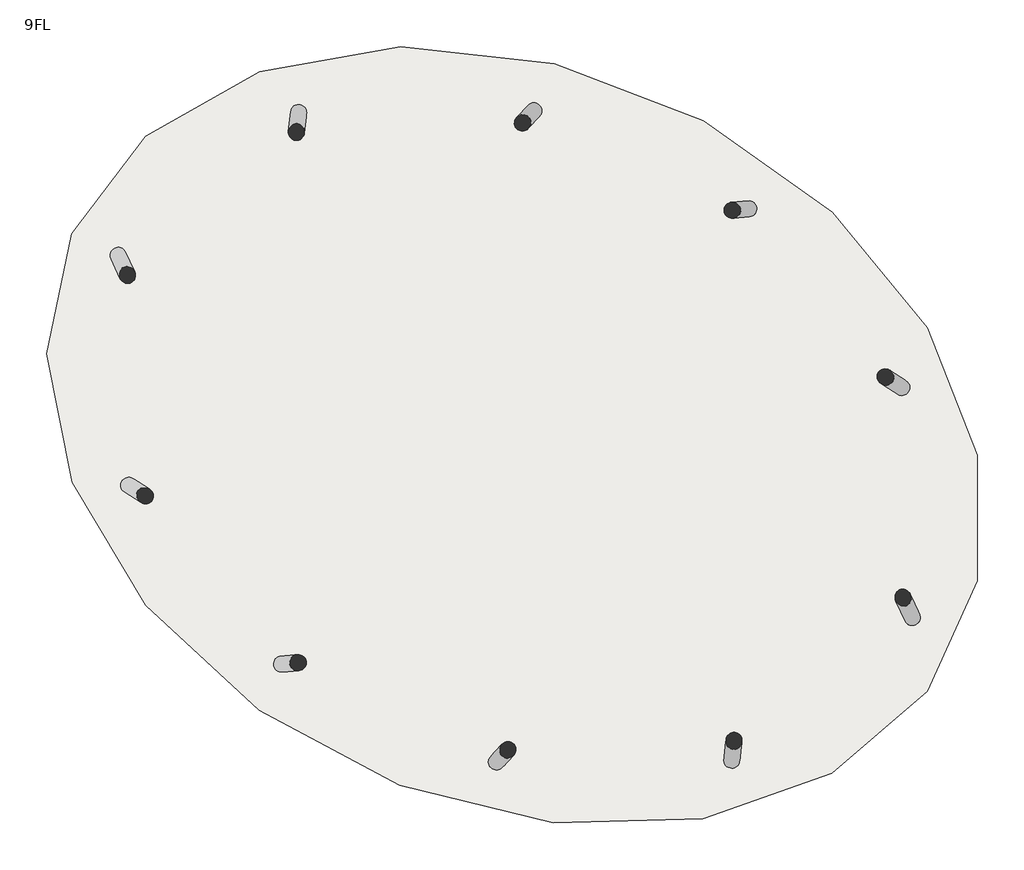
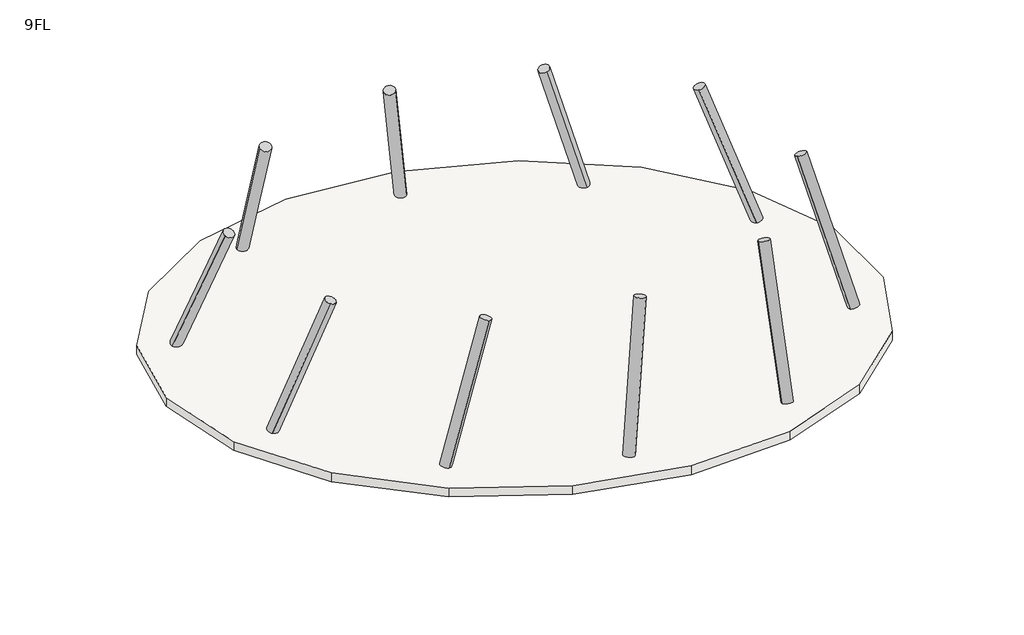
# One storey: 10 columns, 1 slab.
"""IFC4 building model written with IfcOpenShell, lengths in millimetres."""

import ifcopenshell
import ifcopenshell.guid

model = None  # the IFC model being written
_history = None  # IfcOwnerHistory: only IFC2X3 demands one
_inside = {}  # id of a spatial element -> (the spatial element, [elements in it])
_under = {}  # id of a project, library or spatial element -> (it, [spatial elements below it])
_declared = {}  # id of a project -> (the project, [libraries it declares])
_typed = {}  # id of a type object -> (the type object, [elements of that type])
_made_of = {}  # id of a material, layer set ... -> (it, [elements and type objects made of it])


def new_model(schema):
    """Start an empty IFC model of exactly this schema.

    Asked for "IFC4X3", IfcOpenShell would pick the latest addendum, in which some entities
    have other attributes; the version numbers below select the first issue.
    IFC2X3 requires an IfcOwnerHistory on every rooted entity: one is made here for all.
    """
    global model, _history
    if schema == "IFC4X3":
        model = ifcopenshell.file(schema_version=(4, 3, 0, 0))
    else:
        model = ifcopenshell.file(schema=schema)
    _inside.clear()
    _under.clear()
    _declared.clear()
    _typed.clear()
    _made_of.clear()
    _history = None
    if model.schema == "IFC2X3":
        org = make("IfcOrganization", Name="unknown")
        user = make(
            "IfcPersonAndOrganization",
            ThePerson=make("IfcPerson", FamilyName="unknown"),
            TheOrganization=org,
        )
        app = make(
            "IfcApplication",
            ApplicationDeveloper=org,
            Version="unknown",
            ApplicationFullName="unknown",
            ApplicationIdentifier="unknown",
        )
        _history = make(
            "IfcOwnerHistory",
            OwningUser=user,
            OwningApplication=app,
            ChangeAction="ADDED",
            CreationDate=0,
        )
    return model


def make(cls, **values):
    """One entity of the class cls with the attributes given. An attribute that is None is left unset."""
    return model.create_entity(
        cls, **{name: value for name, value in values.items() if value is not None}
    )


def rooted(cls, **values):
    """An entity with a GlobalId (a new one), such as an element, a storey or a relation."""
    return make(cls, GlobalId=ifcopenshell.guid.new(), OwnerHistory=_history, **values)


def si_unit(unit_type, name, prefix=None):
    """IfcSIUnit, for example si_unit("LENGTHUNIT", "METRE", prefix="MILLI")."""
    return make("IfcSIUnit", UnitType=unit_type, Prefix=prefix, Name=name)


def assignment(units):
    """IfcUnitAssignment: the units of a project."""
    return None if units is None else make("IfcUnitAssignment", Units=units)


def point(xyz):
    """IfcCartesianPoint."""
    return None if xyz is None else make("IfcCartesianPoint", Coordinates=xyz)


def direction(xyz):
    """IfcDirection."""
    return None if xyz is None else make("IfcDirection", DirectionRatios=xyz)


def frame(location, z_axis=None, x_axis=None):
    """IfcAxis2Placement3D, a coordinate frame: its origin and axes. An axis left out is left unset."""
    return make(
        "IfcAxis2Placement3D",
        Location=point(location),
        Axis=direction(z_axis),
        RefDirection=direction(x_axis),
    )


def frame_2d(location, x_axis=None):
    """IfcAxis2Placement2D, a coordinate frame in the plane: its origin and x axis."""
    return make(
        "IfcAxis2Placement2D", Location=point(location), RefDirection=direction(x_axis)
    )


def origin():
    """The frame at (0, 0, 0) with its axes left unset."""
    return frame((0.0, 0.0, 0.0))


def place(relative_to, where):
    """IfcLocalPlacement: puts the frame where relative to a parent placement (None: the world)."""
    return make(
        "IfcLocalPlacement", PlacementRelTo=relative_to, RelativePlacement=where
    )


def context(
    kind, dimensions, precision=None, world=None, true_north=None, identifier=None
):
    """IfcGeometricRepresentationContext, for example the 3D "Model" context."""
    return make(
        "IfcGeometricRepresentationContext",
        ContextIdentifier=identifier,
        ContextType=kind,
        CoordinateSpaceDimension=dimensions,
        Precision=precision,
        WorldCoordinateSystem=world,
        TrueNorth=true_north,
    )


def project(units=None, contexts=None):
    """IfcProject with its units and contexts."""
    return rooted(
        "IfcProject",
        Name="project",
        RepresentationContexts=contexts,
        UnitsInContext=assignment(units),
    )


def spatial(cls, under=None, at=None, **own):
    """A site, building, storey or space (cls), placed at a placement, below another one or the project."""
    s = rooted(cls, ObjectPlacement=at, **own)
    if under is not None:
        _under.setdefault(under.id(), (under, []))[1].append(s)
    return s


def polyline(points):
    """IfcPolyline through the points."""
    return make("IfcPolyline", Points=[point(p) for p in points])


def circle_curve(where, radius):
    """IfcCircle in the frame where."""
    return make("IfcCircle", Position=where, Radius=radius)


def trimmed(basis, trim1, trim2, sense, master):
    """IfcTrimmedCurve: the piece of a basis curve between two trims."""
    return make(
        "IfcTrimmedCurve",
        BasisCurve=basis,
        Trim1=trim1,
        Trim2=trim2,
        SenseAgreement=sense,
        MasterRepresentation=master,
    )


def segment(curve, same_sense, transition):
    """IfcCompositeCurveSegment."""
    return make(
        "IfcCompositeCurveSegment",
        Transition=transition,
        SameSense=same_sense,
        ParentCurve=curve,
    )


def composite_curve(segments, self_intersect=None):
    """IfcCompositeCurve: segments joined end to end."""
    return make("IfcCompositeCurve", Segments=segments, SelfIntersect=self_intersect)


def outline(outer, holes=None, kind="AREA"):
    """IfcArbitraryClosedProfileDef: a profile drawn as a closed curve; with holes, ...WithVoids."""
    if holes is None:
        return make("IfcArbitraryClosedProfileDef", ProfileType=kind, OuterCurve=outer)
    return make(
        "IfcArbitraryProfileDefWithVoids",
        ProfileType=kind,
        OuterCurve=outer,
        InnerCurves=holes,
    )


def extrude(swept, where, along, depth):
    """IfcExtrudedAreaSolid: the profile swept, set in the frame where, extruded along a direction by depth."""
    return make(
        "IfcExtrudedAreaSolid",
        SweptArea=swept,
        Position=where,
        ExtrudedDirection=direction(along),
        Depth=depth,
    )


def shape(context_of_items, identifier, shape_type, items):
    """IfcShapeRepresentation: the items that make up one representation, for example the "Body"."""
    return make(
        "IfcShapeRepresentation",
        ContextOfItems=context_of_items,
        RepresentationIdentifier=identifier,
        RepresentationType=shape_type,
        Items=items,
    )


def made_of(thing, what):
    """Note that an element or type object is made of a material, layer set ...; save() writes the relation."""
    if what is not None:
        _made_of.setdefault(what.id(), (what, []))[1].append(thing)
    return thing


def element(
    cls,
    number,
    at=None,
    inside=None,
    cuts=None,
    type_object=None,
    material=None,
    context=None,
    identifier="Body",
    shape_type=None,
    held_by="IfcProductDefinitionShape",
    body=None,
    shapes=None,
    **own,
):
    """One element of the class cls, such as IfcWall. Its Tag is "e" and its number.

    at: its placement. inside: the storey or other place that contains it. cuts: it is an
    opening in that element (IfcRelVoidsElement). A single representation is given by context,
    identifier, shape_type and body (its items); several are given by shapes. held_by: the class
    of the entity that holds the representations. save() writes the other relations.
    """
    e = rooted(cls, Tag="e%d" % number, ObjectPlacement=at, **own)
    if body is not None:
        shapes = [shape(context, identifier, shape_type, body)]
    if shapes is not None:
        e.Representation = make(held_by, Representations=shapes)
    if inside is not None:
        _inside.setdefault(inside.id(), (inside, []))[1].append(e)
    if cuts is not None:
        rooted(
            "IfcRelVoidsElement", RelatingBuildingElement=cuts, RelatedOpeningElement=e
        )
    if type_object is not None:
        _typed.setdefault(type_object.id(), (type_object, []))[1].append(e)
    return made_of(e, material)


def aggregate(whole, parts):
    """IfcRelAggregates: a whole, such as a stair, and the parts it consists of."""
    return rooted("IfcRelAggregates", RelatingObject=whole, RelatedObjects=parts)


def save(model, path):
    """Write the relations noted so far, then the file.

    IfcRelAggregates (storeys below a building ...), IfcRelContainedInSpatialStructure (elements
    in a storey), IfcRelDefinesByType, IfcRelAssociatesMaterial and IfcRelDeclares: one each for
    every whole, place, type object, material and project.
    """
    for whole, parts in _under.values():
        aggregate(whole, parts)
    for where, things in _inside.values():
        rooted(
            "IfcRelContainedInSpatialStructure",
            RelatedElements=things,
            RelatingStructure=where,
        )
    for kind, things in _typed.values():
        rooted("IfcRelDefinesByType", RelatedObjects=things, RelatingType=kind)
    for what, things in _made_of.values():
        rooted("IfcRelAssociatesMaterial", RelatedObjects=things, RelatingMaterial=what)
    for by, libraries in _declared.values():
        rooted("IfcRelDeclares", RelatingContext=by, RelatedDefinitions=libraries)
    model.write(path)


model = new_model("IFC4")

# Units and contexts
model_context = context("Model", 3, world=origin())
ifc_project = project(units=[si_unit("LENGTHUNIT", "METRE", prefix="MILLI")], contexts=[model_context])

# Site, building, storey
site = spatial("IfcSite", under=ifc_project)
building = spatial("IfcBuilding", under=site)
storey = spatial("IfcBuildingStorey", under=building, Name="9FL", Elevation=36000.0)

# Columns
placement = place(None, origin())
element("IfcColumn", 1, ObjectType="コンクリート-円形-柱 : 750", at=placement, inside=storey, context=model_context, shape_type="SweptSolid", body=[
    extrude(outline(composite_curve([segment(trimmed(circle_curve(frame_2d((0.0, -175.0)), 175.0), [point((0.0, -350.0))], [point((0.0, 0.0))], False, "CARTESIAN"), True, "CONTINUOUS"), segment(trimmed(circle_curve(frame_2d((0.0, -175.0)), 175.0), [point((0.0, 0.0))], [point((0.0, -350.0))], False, "CARTESIAN"), True, "CONTINUOUS")], self_intersect=False)), frame((-8514.2452666, 4034.6568807, 36000.0), z_axis=(0.15733612172811792, -0.3378236553256983, 0.9279657982393201), x_axis=(0.39177919901392977, -0.8412072169934959, -0.3726653690619258)), (0.0, 0.0, 1.0), 4849.3166543),
])
element("IfcColumn", 2, ObjectType="コンクリート-円形-柱 : 750", at=placement, inside=storey, context=model_context, shape_type="SweptSolid", body=[
    extrude(outline(composite_curve([segment(trimmed(circle_curve(frame_2d((0.0, -175.0)), 175.0), [point((0.0, -350.0))], [point((0.0, 0.0))], False, "CARTESIAN"), True, "CONTINUOUS"), segment(trimmed(circle_curve(frame_2d((0.0, -175.0)), 175.0), [point((0.0, 0.0))], [point((0.0, -350.0))], False, "CARTESIAN"), True, "CONTINUOUS")], self_intersect=False)), frame((-8350.4905553, -915.6888935, 36000.0), z_axis=(0.2847052316453447, -0.1823560957618653, 0.9411106127402136), x_axis=(0.7924875693780975, -0.5075949544602028, -0.33809882370061567)), (0.0, 0.0, 1.0), 4781.5845864),
])
element("IfcColumn", 3, ObjectType="コンクリート-円形-柱 : 750", at=placement, inside=storey, context=model_context, shape_type="SweptSolid", body=[
    extrude(outline(composite_curve([segment(trimmed(circle_curve(frame_2d((0.0, -175.0)), 175.0), [point((0.0, -350.0))], [point((0.0, 0.0))], False, "CARTESIAN"), True, "CONTINUOUS"), segment(trimmed(circle_curve(frame_2d((0.0, -175.0)), 175.0), [point((0.0, 0.0))], [point((0.0, -350.0))], False, "CARTESIAN"), True, "CONTINUOUS")], self_intersect=False)), frame((-5119.8607282, -4795.3472687, 36000.0), z_axis=(0.28943616732843275, 0.02500202498113821, 0.9568707351513422), x_axis=(0.953320592114223, 0.08234957461977091, -0.2905140206787445)), (0.0, 0.0, 1.0), 4702.8295826),
])
element("IfcColumn", 4, ObjectType="コンクリート-円形-柱 : 750", at=placement, inside=storey, context=model_context, shape_type="SweptSolid", body=[
    extrude(outline(composite_curve([segment(trimmed(circle_curve(frame_2d((-1e-07, -175.0)), 175.0), [point((0.0, -350.0))], [point((0.0, 0.0))], False, "CARTESIAN"), True, "CONTINUOUS"), segment(trimmed(circle_curve(frame_2d((-1e-07, -175.0)), 175.0), [point((0.0, 0.0))], [point((0.0, -350.0))], False, "CARTESIAN"), True, "CONTINUOUS")], self_intersect=False)), frame((-540.8791395, -6993.0373968, 36000.0), z_axis=(0.19954005269082362, 0.21390210923148706, 0.9562581529265328), x_axis=(0.6522943128916165, 0.6992437231807793, -0.29252409295908555)), (0.0, 0.0, 1.0), 4705.8422299),
])
element("IfcColumn", 5, ObjectType="コンクリート-円形-柱 : 750", at=placement, inside=storey, context=model_context, shape_type="SweptSolid", body=[
    extrude(outline(composite_curve([segment(trimmed(circle_curve(frame_2d((0.0, -175.0)), 175.0), [point((0.0, -350.0))], [point((0.0, 0.0))], False, "CARTESIAN"), True, "CONTINUOUS"), segment(trimmed(circle_curve(frame_2d((0.0, -175.0)), 175.0), [point((0.0, 0.0))], [point((0.0, -350.0))], False, "CARTESIAN"), True, "CONTINUOUS")], self_intersect=False)), frame((4552.9597741, -7058.4040402, 36000.0), z_axis=(0.038876985986662435, 0.3386274609145675, 0.9401170260532175), x_axis=(0.10722816215418955, 0.9339818755822732, -0.34085184072387537)), (0.0, 0.0, 1.0), 4786.6381274),
])
element("IfcColumn", 6, ObjectType="コンクリート-円形-柱 : 750", at=placement, inside=storey, context=model_context, shape_type="SweptSolid", body=[
    extrude(outline(composite_curve([segment(trimmed(circle_curve(frame_2d((0.0, -175.0)), 175.0), [point((1e-07, -350.0))], [point((0.0, 0.0))], False, "CARTESIAN"), True, "CONTINUOUS"), segment(trimmed(circle_curve(frame_2d((0.0, -175.0)), 175.0), [point((0.0, 0.0))], [point((1e-07, -350.0))], False, "CARTESIAN"), True, "CONTINUOUS")], self_intersect=False)), frame((8514.2452947, -4034.656857, 36000.0), z_axis=(-0.15733612285483128, 0.3378236560647704, 0.9279657977792293), x_axis=(-0.3917792004208642, 0.841207215830695, -0.3726653702075883)), (0.0, 0.0, 1.0), 4849.3166543),
])
element("IfcColumn", 7, ObjectType="コンクリート-円形-柱 : 750", at=placement, inside=storey, context=model_context, shape_type="SweptSolid", body=[
    extrude(outline(composite_curve([segment(trimmed(circle_curve(frame_2d((0.0, -175.0)), 175.0), [point((0.0, -350.0))], [point((0.0, 0.0))], False, "CARTESIAN"), True, "CONTINUOUS"), segment(trimmed(circle_curve(frame_2d((0.0, -175.0)), 175.0), [point((0.0, 0.0))], [point((0.0, -350.0))], False, "CARTESIAN"), True, "CONTINUOUS")], self_intersect=False)), frame((8350.4905214, 915.6889185, 36000.0), z_axis=(-0.2847052323966988, 0.18235609172631548, 0.9411106132948694), x_axis=(-0.7924875755554238, 0.5075949458441562, -0.3380988221567101)), (0.0, 0.0, 1.0), 4781.5845864),
])
element("IfcColumn", 8, ObjectType="コンクリート-円形-柱 : 750", at=placement, inside=storey, context=model_context, shape_type="SweptSolid", body=[
    extrude(outline(composite_curve([segment(trimmed(circle_curve(frame_2d((0.0, -175.0)), 175.0), [point((0.0, -350.0))], [point((0.0, 0.0))], False, "CARTESIAN"), True, "CONTINUOUS"), segment(trimmed(circle_curve(frame_2d((0.0, -175.0)), 175.0), [point((0.0, 0.0))], [point((0.0, -350.0))], False, "CARTESIAN"), True, "CONTINUOUS")], self_intersect=False)), frame((5119.8606888, 4795.3472775, 36000.0), z_axis=(-0.2894361653262684, -0.025002027929639317, 0.9568707356799196), x_axis=(-0.9533205917593104, -0.0823495848702891, -0.29051401893776047)), (0.0, 0.0, 1.0), 4702.8295826),
])
element("IfcColumn", 9, ObjectType="コンクリート-円形-柱 : 750", at=placement, inside=storey, context=model_context, shape_type="SweptSolid", body=[
    extrude(outline(composite_curve([segment(trimmed(circle_curve(frame_2d((-1e-07, -175.0)), 175.0), [point((0.0, -350.0))], [point((0.0, 0.0))], False, "CARTESIAN"), True, "CONTINUOUS"), segment(trimmed(circle_curve(frame_2d((-1e-07, -175.0)), 175.0), [point((0.0, 0.0))], [point((0.0, -350.0))], False, "CARTESIAN"), True, "CONTINUOUS")], self_intersect=False)), frame((540.8791451, 6993.0373957, 36000.0), z_axis=(-0.19954005506216624, -0.21390210898903245, 0.9562581524859446), x_axis=(-0.6522943171313185, -0.6992437186232128, -0.29252409439936433)), (0.0, 0.0, 1.0), 4705.8422299),
])
element("IfcColumn", 10, ObjectType="コンクリート-円形-柱 : 750", at=placement, inside=storey, context=model_context, shape_type="SweptSolid", body=[
    extrude(outline(composite_curve([segment(trimmed(circle_curve(frame_2d((1e-07, -175.0)), 175.0), [point((0.0, -350.0))], [point((0.0, 0.0))], False, "CARTESIAN"), True, "CONTINUOUS"), segment(trimmed(circle_curve(frame_2d((1e-07, -175.0)), 175.0), [point((0.0, 0.0))], [point((0.0, -350.0))], False, "CARTESIAN"), True, "CONTINUOUS")], self_intersect=False)), frame((-4552.9597594, 7058.4040637, 36000.0), z_axis=(-0.03887699228619042, -0.33862746155916207, 0.9401170255605299), x_axis=(-0.10722817904547799, -0.9339818731471016, -0.34085184208277686)), (0.0, 0.0, 1.0), 4786.6381274),
])

# Slab
element("IfcSlab", 11, ObjectType="一般 300 mm", at=placement, inside=storey, context=model_context, shape_type="SweptSolid", body=[
    extrude(outline(polyline([(-9672.5882037, -997.2978672), (-10231.1139666, 1806.150389), (-9675.7034427, 4418.7457038), (-8064.952189, 6549.3830561), (-5580.4907716, 7963.1456311), (-2496.7389426, 8511.1496001), (853.1543364, 8139.231312), (4109.7885929, 6889.8255974), (6923.7341951, 4897.4913273), (8992.0881279, 2374.9256891), (10089.6813215, -409.1203495), (10092.0644821, -3155.2925015), (8993.5077014, -5560.7962627), (6916.5286541, -7357.3555199), (4093.7163534, -8351.0123567), (832.8046727, -8439.7839579), (-2515.6435878, -7617.8472233), (-5592.5233278, -5974.834021), (-8067.313984, -3686.7082806), (-9672.5882037, -997.2978672)])), frame((0.0, 0.0, 35700.0), z_axis=(0.0, 0.0, 1.0), x_axis=(1.0, 0.0, 0.0)), (0.0, 0.0, 1.0), 300.0),
])

save(model, "model.ifc")

# Revit data of these elements
# Type "コンクリート-円形-柱 : 750"
#   Keynote = "03310.Q1"
#   R = 350 mm
#   Structural Material [instance default] = コンクリート - 現場打ち
# Type "一般 300 mm"
#   Function = 0
#   Layers, outside or top first: 300 mm no material (function 1)
# Elements 1, 2, 3, 4, 5, 6, 7, 8, 9, 10 (IfcColumn, "コンクリート-円形-柱 : 750")
#   Structural Material = コンクリート - 現場打ち
#   Phase Created = 新しい建設
#   Materials on its faces: "コンクリート - 現場打ち"
# Element 11 (IfcSlab, "一般 300 mm")
#   Height Offset From Level = 0 mm
#   Phase Created = 新しい建設
# Materials
#   "コンクリート - 現場打ち": class "コンクリート", colour RGB 192 192 192, transparency 0
